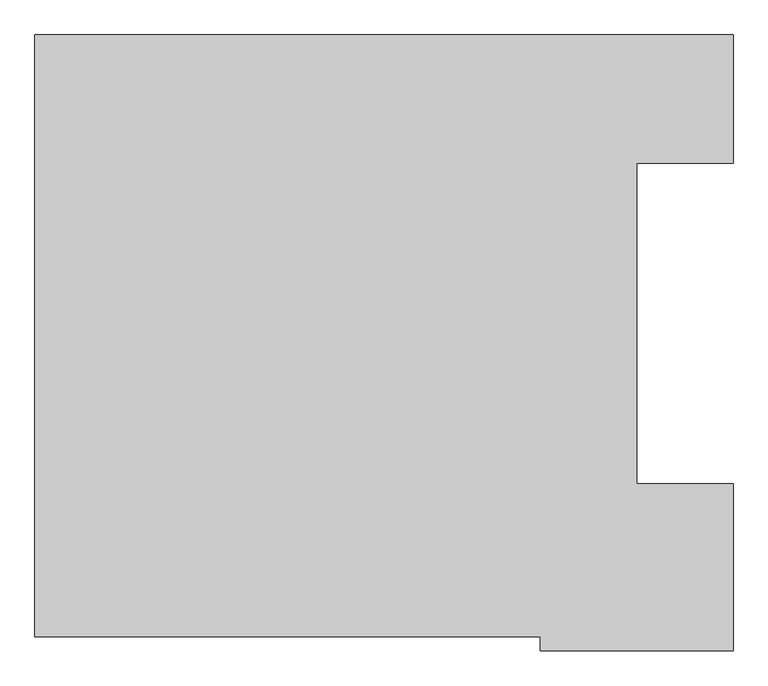
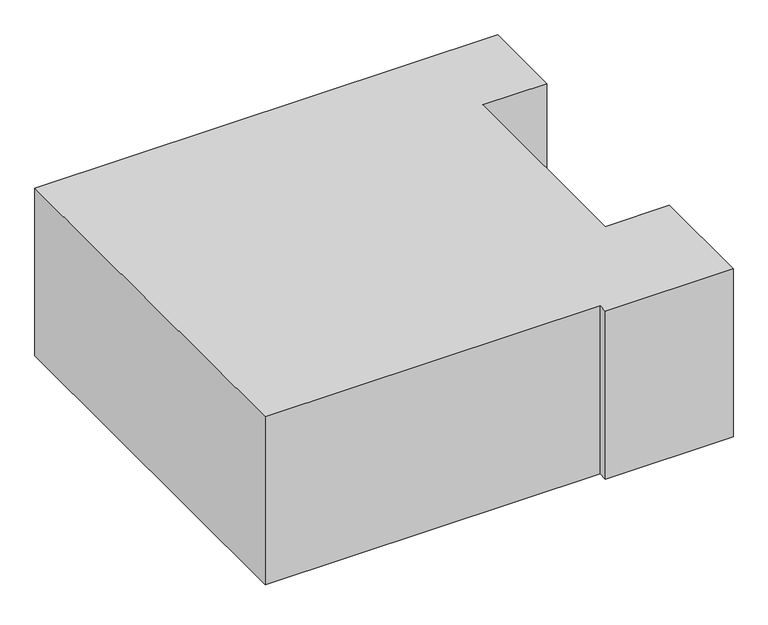
"""IFC4 building model written with IfcOpenShell, lengths in millimetres: proxy geometry, 0_3d."""

from ifc_helpers import new_model, si_unit, origin, origin_with_axes, place, context, project, spatial, polyline, outline, extrude, source, transform, mapped, element, save


def generic_models_0361ec3a(model_context):
    return source(origin(), model_context, "Body", "SweptSolid", [
        extrude(outline(polyline([(6520.0, 0.0), (4720.0, 0.0), (4720.0, 130.0), (0.0, 130.0), (0.0, 5750.0), (6520.0, 5750.0), (6520.0, 4550.0), (5620.0, 4550.0), (5620.0, 1560.0), (6520.0, 1560.0), (6520.0, 0.0)])), origin_with_axes(), (0.0, 0.0, 1.0), 2500.0),
    ])


if __name__ == "__main__":
    model = new_model("IFC4")
    model_context = context("Model", 3, world=origin())
    ifc_project = project(units=[si_unit("LENGTHUNIT", "METRE", prefix="MILLI")], contexts=[model_context])
    site = spatial("IfcSite", under=ifc_project)
    building = spatial("IfcBuilding", under=site)
    placement = place(None, origin())
    generic_models_shape = generic_models_0361ec3a(model_context)
    element("IfcBuildingElementProxy", 1, Name="0_3d", ObjectType="0_3d", at=placement, inside=building, context=model_context, shape_type="MappedRepresentation", body=[
        mapped(generic_models_shape, transform((0.0, 0.0, 0.0), x_axis=(1.0, 0.0, 0.0), y_axis=(0.0, 1.0, 0.0), z_axis=(0.0, 0.0, 1.0))),
    ])
    save(model, "model.ifc")

# Revit data of these elements
# Project information
#   Organization Name = "Organization Name"
#   Organization Description = "Organization Description"
#   Building Name = "Building Name"
#   IfcOrganization = "KURIARCHITEKTEN"
#   IfcApplicationVersion = "2023.1"
#   IfcApplicationName = "Allplan"
#   IfcSite GUID = "3xMs$kp1n46ejeur8tozco"
#   IfcBuilding GUID = "0i8UyhEYT3nv9HLlo1H2X7"
#   IfcProject GUID = "2x1YFttxr4OvBiL8xtaqeA"
#   IfcDecomposes = "BVH Tammik Wohnhaus Waldrain"
#   IfcDecomposesGUID = "2x1YFttxr4OvBiL8xtaqeA"
#   IfcPropertySetList = "\"AllplanAttributes\""
#   BuildingName = "GEBÄUDE 1"
#   SiteName = "BAUANTRAG"
#   IfcProject Name = "BVH Tammik Wohnhaus Waldrain"
#   AllplanAttributes.Land = "IFC - Land"
#   AllplanAttributes.Bundesland = "IFC - Bundesland"
#   AllplanAttributes.Prüfer = "Prüfstatiker"
#   AllplanAttributes.Bauherr = "Jeremy Tammik"
#   AllplanAttributes.Bruttogeschossfläche = "IFC - Bruttogeschossfläche"
#   AllplanAttributes.Projektleiter = "Projektleitername"
#   AllplanAttributes.Architekt = "Architektenname"
#   AllplanAttributes.Statik = "Statiker"
#   AllplanAttributes.Elektro = "Elektroplaner"
#   AllplanAttributes.Heizung = "Heizungsplaner"
#   AllplanAttributes.Sanitär = "Sanitärplaner"
#   AllplanAttributes.Bebaubare Fläche = "IFC - bebaubare Fläche"
#   AllplanAttributes.Maximale Gebäudehöhe = "IFC - Maximale Gebäudehöhe"
#   AllplanAttributes.Bruttogrundstücksfläche = "IFC - Bruttogrundstücksfläche"
#   AllplanAttributes.Normalhöhennull = "IFC - Höhe über NN"
#   AllplanAttributes.Projektvorlage = "IBD 2023"
#   AllplanAttributes.Bauvorhaben = "BVH Waldrain"
#   AllplanAttributes.Bauherr Straße = "Hühnerbergweg 30"
#   AllplanAttributes.Bauherr Plz/Ort = "79539 Lörrach"
#   AllplanAttributes.Architekt Straße = "Architektenstrasse 111"
#   AllplanAttributes.Architekt Plz/Ort = "72108 Architektenort"
#   AllplanAttributes.Bauvorhaben Straße = "Carl-Keller-Weg 6"
#   AllplanAttributes.Bauvorhaben Plz/Ort = "79539 Lörrach"
#   AllplanAttributes.Projektnummer = "2023"
#   AllplanAttributes.Architekt Telefonnummer = "07472-93791-0"
#   AllplanAttributes.Architekt Telefaxnummer = "07472/93791-29"
#   AllplanAttributes.Projektbeschreibung = "Projektnamen Ergänzung"
#   AllplanAttributes.Geographische Länge = "IFC - Geografische Länge"
#   AllplanAttributes.Geographische Breite = "IFC - Geografische Breite"
#   AllplanAttributes.Architekt E-Mail = "Architekt@email.de"
#   Original IFC File Name = "Y:\\j\\doc\\house\\huenerberg\\waldrain\\html\\waldrain.github.io\\doc\\biz\\kuri\\2024-02-21\\0_3d.ifc"
#   Original IFC File Size = "5603191"
#   Revit File Last Updated = "638441278712508807"
#   Revit Importer Version = "Importer 24.2.0.63"
#   Import Method = "Hybrid"
#   Project Issue Date = "Issue Date"
#   Project Status = "Project Status"
#   Client Name = "Client Name"
#   Project Address = "Enter address here\nAddress Line 2"
#   Project Name = "Project Name"
#   Project Number = "Project Number"
# Element 1 (IfcBuildingElementProxy, "0_3d")
#   Materials on its faces: "*1"
# Materials
#   "*1": class "Unassigned", colour RGB 175 175 175, transparency 0
